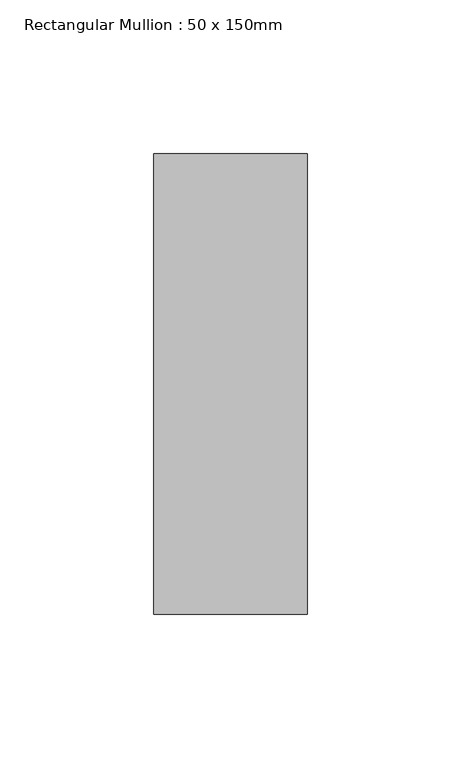
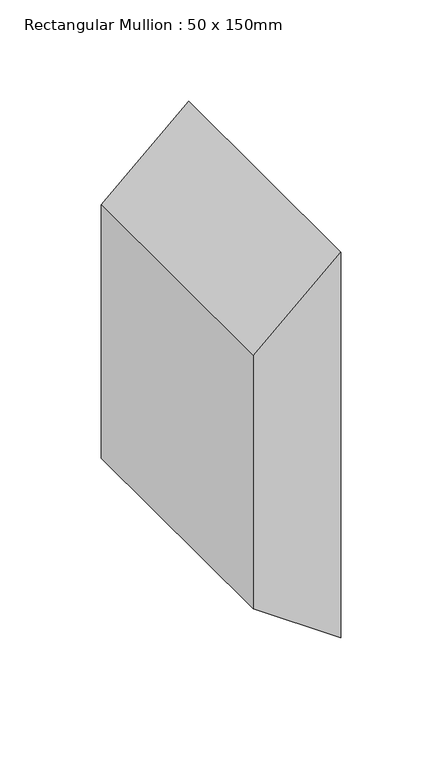
"""IFC4 building model written with IfcOpenShell, lengths in millimetres: member geometry, Rectangular Mullion : 50 x 150mm."""

from ifc_helpers import new_model, si_unit, frame, origin, place, context, project, spatial, polyline, outline, extrude, source, transform, mapped, element, save


def rectangular_mullion_50_x_150mm_55f3bd26(model_context):
    return source(origin(), model_context, "Body", "SweptSolid", [
        extrude(outline(polyline([(0.0, 0.0), (-44.8446171, -50.0), (-197.6121942, -50.0), (-232.5177317, 0.0), (0.0, 0.0)])), frame((0.0, -75.0, 0.0), z_axis=(0.0, 1.0, 0.0), x_axis=(0.0, 0.0, 1.0)), (0.0, 0.0, 1.0), 150.0),
    ])


if __name__ == "__main__":
    model = new_model("IFC4")
    model_context = context("Model", 3, world=origin())
    ifc_project = project(units=[si_unit("LENGTHUNIT", "METRE", prefix="MILLI")], contexts=[model_context])
    site = spatial("IfcSite", under=ifc_project)
    building = spatial("IfcBuilding", under=site)
    placement = place(None, origin())
    rectangular_mullion_50_x_150mm_shape = rectangular_mullion_50_x_150mm_55f3bd26(model_context)
    element("IfcMember", 1, ObjectType="Rectangular Mullion : 50 x 150mm", at=placement, inside=building, context=model_context, shape_type="MappedRepresentation", body=[
        mapped(rectangular_mullion_50_x_150mm_shape, transform((0.0, 0.0, 0.0), x_axis=(1.0, 0.0, 0.0), y_axis=(0.0, 1.0, 0.0), z_axis=(0.0, 0.0, 1.0))),
    ])
    save(model, "model.ifc")

# Revit data of these elements
# Type "Rectangular Mullion : 50 x 150mm"
#   built-in parameter 1007304 = 0.492126 (stored number, unit not read)
#   built-in parameter 1007301 = 0.082021 (stored number, unit not read)
#   built-in parameter 1007300 = 0.082021 (stored number, unit not read)
# Element 1 (IfcMember, "Rectangular Mullion : 50 x 150mm")
#   Materials on its faces: "Metal - Aluminium"
# Materials
#   "Metal - Aluminium": class "Metal", colour RGB 247 247 247, transparency 0
